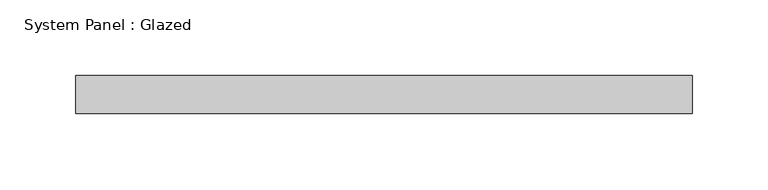
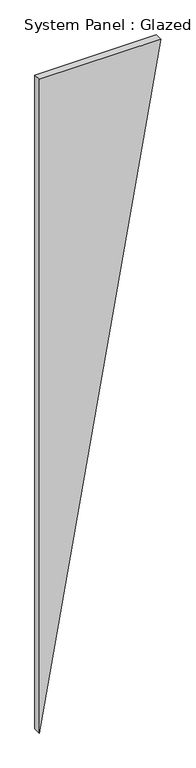
"""IFC4 building model written with IfcOpenShell, lengths in millimetres: plate geometry, System Panel : Glazed."""

import ifcopenshell
import ifcopenshell.guid

model = None  # the IFC model being written
_history = None  # IfcOwnerHistory: only IFC2X3 demands one
_inside = {}  # id of a spatial element -> (the spatial element, [elements in it])
_under = {}  # id of a project, library or spatial element -> (it, [spatial elements below it])
_declared = {}  # id of a project -> (the project, [libraries it declares])
_typed = {}  # id of a type object -> (the type object, [elements of that type])
_made_of = {}  # id of a material, layer set ... -> (it, [elements and type objects made of it])


def new_model(schema):
    """Start an empty IFC model of exactly this schema.

    Asked for "IFC4X3", IfcOpenShell would pick the latest addendum, in which some entities
    have other attributes; the version numbers below select the first issue.
    IFC2X3 requires an IfcOwnerHistory on every rooted entity: one is made here for all.
    """
    global model, _history
    if schema == "IFC4X3":
        model = ifcopenshell.file(schema_version=(4, 3, 0, 0))
    else:
        model = ifcopenshell.file(schema=schema)
    _inside.clear()
    _under.clear()
    _declared.clear()
    _typed.clear()
    _made_of.clear()
    _history = None
    if model.schema == "IFC2X3":
        org = make("IfcOrganization", Name="unknown")
        user = make(
            "IfcPersonAndOrganization",
            ThePerson=make("IfcPerson", FamilyName="unknown"),
            TheOrganization=org,
        )
        app = make(
            "IfcApplication",
            ApplicationDeveloper=org,
            Version="unknown",
            ApplicationFullName="unknown",
            ApplicationIdentifier="unknown",
        )
        _history = make(
            "IfcOwnerHistory",
            OwningUser=user,
            OwningApplication=app,
            ChangeAction="ADDED",
            CreationDate=0,
        )
    return model


def make(cls, **values):
    """One entity of the class cls with the attributes given. An attribute that is None is left unset."""
    return model.create_entity(
        cls, **{name: value for name, value in values.items() if value is not None}
    )


def rooted(cls, **values):
    """An entity with a GlobalId (a new one), such as an element, a storey or a relation."""
    return make(cls, GlobalId=ifcopenshell.guid.new(), OwnerHistory=_history, **values)


def si_unit(unit_type, name, prefix=None):
    """IfcSIUnit, for example si_unit("LENGTHUNIT", "METRE", prefix="MILLI")."""
    return make("IfcSIUnit", UnitType=unit_type, Prefix=prefix, Name=name)


def assignment(units):
    """IfcUnitAssignment: the units of a project."""
    return None if units is None else make("IfcUnitAssignment", Units=units)


def point(xyz):
    """IfcCartesianPoint."""
    return None if xyz is None else make("IfcCartesianPoint", Coordinates=xyz)


def direction(xyz):
    """IfcDirection."""
    return None if xyz is None else make("IfcDirection", DirectionRatios=xyz)


def frame(location, z_axis=None, x_axis=None):
    """IfcAxis2Placement3D, a coordinate frame: its origin and axes. An axis left out is left unset."""
    return make(
        "IfcAxis2Placement3D",
        Location=point(location),
        Axis=direction(z_axis),
        RefDirection=direction(x_axis),
    )


def origin():
    """The frame at (0, 0, 0) with its axes left unset."""
    return frame((0.0, 0.0, 0.0))


def place(relative_to, where):
    """IfcLocalPlacement: puts the frame where relative to a parent placement (None: the world)."""
    return make(
        "IfcLocalPlacement", PlacementRelTo=relative_to, RelativePlacement=where
    )


def context(
    kind, dimensions, precision=None, world=None, true_north=None, identifier=None
):
    """IfcGeometricRepresentationContext, for example the 3D "Model" context."""
    return make(
        "IfcGeometricRepresentationContext",
        ContextIdentifier=identifier,
        ContextType=kind,
        CoordinateSpaceDimension=dimensions,
        Precision=precision,
        WorldCoordinateSystem=world,
        TrueNorth=true_north,
    )


def project(units=None, contexts=None):
    """IfcProject with its units and contexts."""
    return rooted(
        "IfcProject",
        Name="project",
        RepresentationContexts=contexts,
        UnitsInContext=assignment(units),
    )


def spatial(cls, under=None, at=None, **own):
    """A site, building, storey or space (cls), placed at a placement, below another one or the project."""
    s = rooted(cls, ObjectPlacement=at, **own)
    if under is not None:
        _under.setdefault(under.id(), (under, []))[1].append(s)
    return s


def polyline(points):
    """IfcPolyline through the points."""
    return make("IfcPolyline", Points=[point(p) for p in points])


def outline(outer, holes=None, kind="AREA"):
    """IfcArbitraryClosedProfileDef: a profile drawn as a closed curve; with holes, ...WithVoids."""
    if holes is None:
        return make("IfcArbitraryClosedProfileDef", ProfileType=kind, OuterCurve=outer)
    return make(
        "IfcArbitraryProfileDefWithVoids",
        ProfileType=kind,
        OuterCurve=outer,
        InnerCurves=holes,
    )


def extrude(swept, where, along, depth):
    """IfcExtrudedAreaSolid: the profile swept, set in the frame where, extruded along a direction by depth."""
    return make(
        "IfcExtrudedAreaSolid",
        SweptArea=swept,
        Position=where,
        ExtrudedDirection=direction(along),
        Depth=depth,
    )


def shape(context_of_items, identifier, shape_type, items):
    """IfcShapeRepresentation: the items that make up one representation, for example the "Body"."""
    return make(
        "IfcShapeRepresentation",
        ContextOfItems=context_of_items,
        RepresentationIdentifier=identifier,
        RepresentationType=shape_type,
        Items=items,
    )


def source(mapping_origin, context_of_items, identifier, shape_type, items):
    """IfcRepresentationMap: a shape defined once, which mapped items show again and again."""
    return make(
        "IfcRepresentationMap",
        MappingOrigin=mapping_origin,
        MappedRepresentation=shape(context_of_items, identifier, shape_type, items),
    )


def transform(
    local_origin,
    x_axis=None,
    y_axis=None,
    z_axis=None,
    scale=None,
    scale2=None,
    scale3=None,
    uniform=True,
):
    """IfcCartesianTransformationOperator3D, or its non-uniform kind. x_axis, y_axis, z_axis: its Axis1, 2, 3."""
    if uniform:
        return make(
            "IfcCartesianTransformationOperator3D",
            Axis1=direction(x_axis),
            Axis2=direction(y_axis),
            LocalOrigin=point(local_origin),
            Scale=scale,
            Axis3=direction(z_axis),
        )
    return make(
        "IfcCartesianTransformationOperator3DnonUniform",
        Axis1=direction(x_axis),
        Axis2=direction(y_axis),
        LocalOrigin=point(local_origin),
        Scale=scale,
        Axis3=direction(z_axis),
        Scale2=scale2,
        Scale3=scale3,
    )


def mapped(mapping_source, mapping_target):
    """IfcMappedItem: shows the shape of a source again, moved by a transform."""
    return make(
        "IfcMappedItem", MappingSource=mapping_source, MappingTarget=mapping_target
    )


def made_of(thing, what):
    """Note that an element or type object is made of a material, layer set ...; save() writes the relation."""
    if what is not None:
        _made_of.setdefault(what.id(), (what, []))[1].append(thing)
    return thing


def element(
    cls,
    number,
    at=None,
    inside=None,
    cuts=None,
    type_object=None,
    material=None,
    context=None,
    identifier="Body",
    shape_type=None,
    held_by="IfcProductDefinitionShape",
    body=None,
    shapes=None,
    **own,
):
    """One element of the class cls, such as IfcWall. Its Tag is "e" and its number.

    at: its placement. inside: the storey or other place that contains it. cuts: it is an
    opening in that element (IfcRelVoidsElement). A single representation is given by context,
    identifier, shape_type and body (its items); several are given by shapes. held_by: the class
    of the entity that holds the representations. save() writes the other relations.
    """
    e = rooted(cls, Tag="e%d" % number, ObjectPlacement=at, **own)
    if body is not None:
        shapes = [shape(context, identifier, shape_type, body)]
    if shapes is not None:
        e.Representation = make(held_by, Representations=shapes)
    if inside is not None:
        _inside.setdefault(inside.id(), (inside, []))[1].append(e)
    if cuts is not None:
        rooted(
            "IfcRelVoidsElement", RelatingBuildingElement=cuts, RelatedOpeningElement=e
        )
    if type_object is not None:
        _typed.setdefault(type_object.id(), (type_object, []))[1].append(e)
    return made_of(e, material)


def aggregate(whole, parts):
    """IfcRelAggregates: a whole, such as a stair, and the parts it consists of."""
    return rooted("IfcRelAggregates", RelatingObject=whole, RelatedObjects=parts)


def save(model, path):
    """Write the relations noted so far, then the file.

    IfcRelAggregates (storeys below a building ...), IfcRelContainedInSpatialStructure (elements
    in a storey), IfcRelDefinesByType, IfcRelAssociatesMaterial and IfcRelDeclares: one each for
    every whole, place, type object, material and project.
    """
    for whole, parts in _under.values():
        aggregate(whole, parts)
    for where, things in _inside.values():
        rooted(
            "IfcRelContainedInSpatialStructure",
            RelatedElements=things,
            RelatingStructure=where,
        )
    for kind, things in _typed.values():
        rooted("IfcRelDefinesByType", RelatedObjects=things, RelatingType=kind)
    for what, things in _made_of.values():
        rooted("IfcRelAssociatesMaterial", RelatedObjects=things, RelatingMaterial=what)
    for by, libraries in _declared.values():
        rooted("IfcRelDeclares", RelatingContext=by, RelatedDefinitions=libraries)
    model.write(path)


def system_panel_glazed_96c5221b(model_context):
    return source(origin(), model_context, "Body", "SweptSolid", [
        extrude(outline(polyline([(0.0, -204.2314386), (2325.3567738, 204.2314386), (2325.3567738, -204.2314386), (0.0, -204.2314386)])), frame((0.0, -44.45, 0.0), z_axis=(0.0, 1.0, 0.0), x_axis=(0.0, 0.0, 1.0)), (0.0, 0.0, 1.0), 25.4),
    ])


if __name__ == "__main__":
    model = new_model("IFC4")
    model_context = context("Model", 3, world=origin())
    ifc_project = project(units=[si_unit("LENGTHUNIT", "METRE", prefix="MILLI")], contexts=[model_context])
    site = spatial("IfcSite", under=ifc_project)
    building = spatial("IfcBuilding", under=site)
    placement = place(None, origin())
    system_panel_glazed_shape = system_panel_glazed_96c5221b(model_context)
    element("IfcPlate", 1, ObjectType="System Panel : Glazed", at=placement, inside=building, context=model_context, shape_type="MappedRepresentation", body=[
        mapped(system_panel_glazed_shape, transform((0.0, 0.0, 0.0), x_axis=(1.0, 0.0, 0.0), y_axis=(0.0, 1.0, 0.0), z_axis=(0.0, 0.0, 1.0))),
    ])
    save(model, "model.ifc")

# Revit data of these elements
# Type "System Panel : Glazed"
#   Construction Type Id = "GSP4R"
#   Analytic Construction = "1/8 in Pilkington single glazing"
#   Visual Light Transmittance = 0.9
#   Solar Heat Gain Coefficient = 0.86
#   Heat Transfer Coefficient (U) = 1.18115 BTU/(h·ft²·°F)
#   Define Thermal Properties by = 1
# Element 1 (IfcPlate, "System Panel : Glazed")
#   Materials on its faces: "Glass"
# Materials
#   "Glass": class "Glass", colour RGB 0 128 192, transparency 0.75, Description = "Soda Lime Glass", Cost = 0
